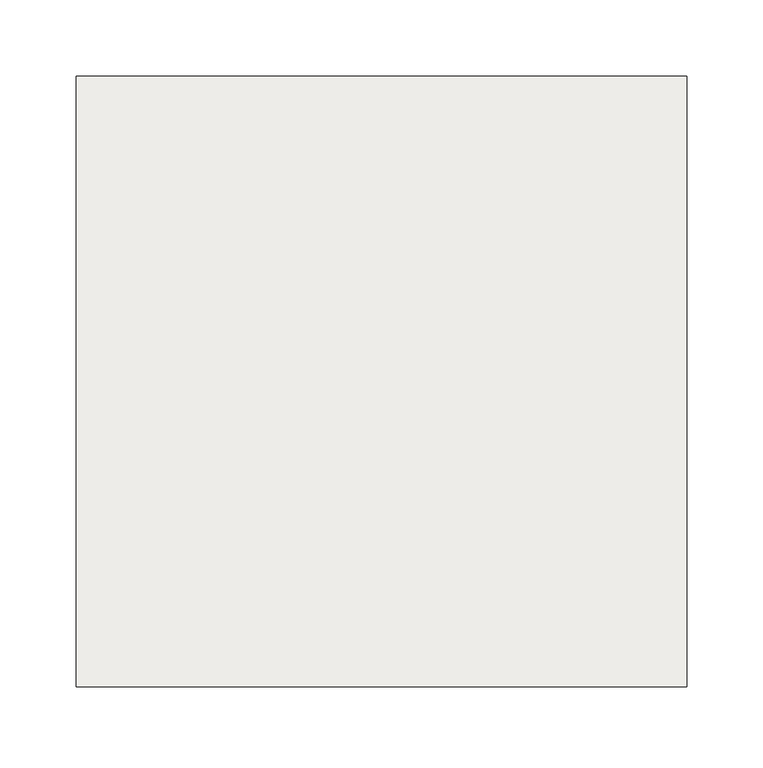
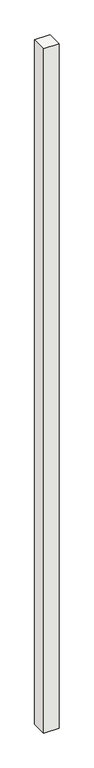
"""IFC4 building model written with IfcOpenShell, lengths in millimetres: slab geometry, NLRS_17_SFO_TLB_funderingspaal geheid beton prefab-AV-MMBPC_gen_rsf : heipaal beton prefab_gen__bxh 400x400."""

from ifc_helpers import new_model, si_unit, frame, origin, place, context, project, spatial, polyline, outline, extrude, source, transform, mapped, element, save


def slab_c87ae41e(model_context):
    return source(origin(), model_context, "Body", "SweptSolid", [
        extrude(outline(polyline([(200.0, -200.0), (-200.0, -200.0), (-200.0, 200.0), (200.0, 200.0), (200.0, -200.0)])), frame((0.0, 0.0, -20000.0), z_axis=(0.0, 0.0, 1.0), x_axis=(1.0, 0.0, 0.0)), (0.0, 0.0, 1.0), 18830.0),
    ])


if __name__ == "__main__":
    model = new_model("IFC4")
    model_context = context("Model", 3, world=origin())
    ifc_project = project(units=[si_unit("LENGTHUNIT", "METRE", prefix="MILLI")], contexts=[model_context])
    site = spatial("IfcSite", under=ifc_project)
    building = spatial("IfcBuilding", under=site)
    placement = place(None, origin())
    slab_shape = slab_c87ae41e(model_context)
    element("IfcSlab", 1, ObjectType="NLRS_17_SFO_TLB_funderingspaal geheid beton prefab-AV-MMBPC_gen_rsf : heipaal beton prefab_gen__bxh 400x400", at=placement, inside=building, context=model_context, shape_type="MappedRepresentation", body=[
        mapped(slab_shape, transform((0.0, 0.0, 0.0), x_axis=(1.0, 0.0, 0.0), y_axis=(0.0, 1.0, 0.0), z_axis=(0.0, 0.0, 1.0))),
    ])
    save(model, "model.ifc")

# Revit data of these elements
# Type "NLRS_17_SFO_TLB_funderingspaal geheid beton prefab-AV-MMBPC_gen_rsf : heipaal beton prefab_gen__bxh 400x400"
#   Export Type to IFC As = "IfcPile"
#   Type IfcGUID = "10$Kfo5uPCAOPJEOo5LE_W"
#   Type Comments = "prefab heipaal 400x400"
#   Model = " "
#   Manufacturer = " "
#   Description = "prefab heipaal 400x400"
#   Assembly Code = "17.21"
#   Width = 400 mm
#   Slanted Angle [instance default] = 0.00°
#   NLRS_S_draagvermogen_trek [instance default] = 0.00 kN
#   NLRS_S_draagvermogen_druk [instance default] = 0.00 kN
#   NLRS_C_lengte [instance default] = 1660 mm
#   NLRS_C_hoogte = 400 mm
#   NLRS_C_breedte = 400 mm
#   Height [instance default] = 1660 mm
#   Length [instance default] = 1660 mm
#   Angle [instance default] = 0.00°
#   Slanted [instance default] = 0
#   Structural Material = NLRS_f2_beton prefab_gen_rsf
#   Keynote = ""
# Element 1 (IfcSlab, "NLRS_17_SFO_TLB_funderingspaal geheid beton prefab-AV-MMBPC_gen_rsf : heipaal beton prefab_gen__bxh 400x400")
#   NLRS_C_lengte = 18830 mm
#   Height = 18830 mm
#   Length = 18830 mm
#   Materials on its faces: "NLRS_f2_beton prefab_gen_rsf"
# Materials
#   "NLRS_f2_beton prefab_gen_rsf": class "F - Niet gebakken kunststeen", colour RGB 129 133 118, transparency 0, Keynote = "f2", Manufacturer = "Revit Standards Foundation", URL = "www.revitstandards.org", Description = "beton prefab", Cost = 0
